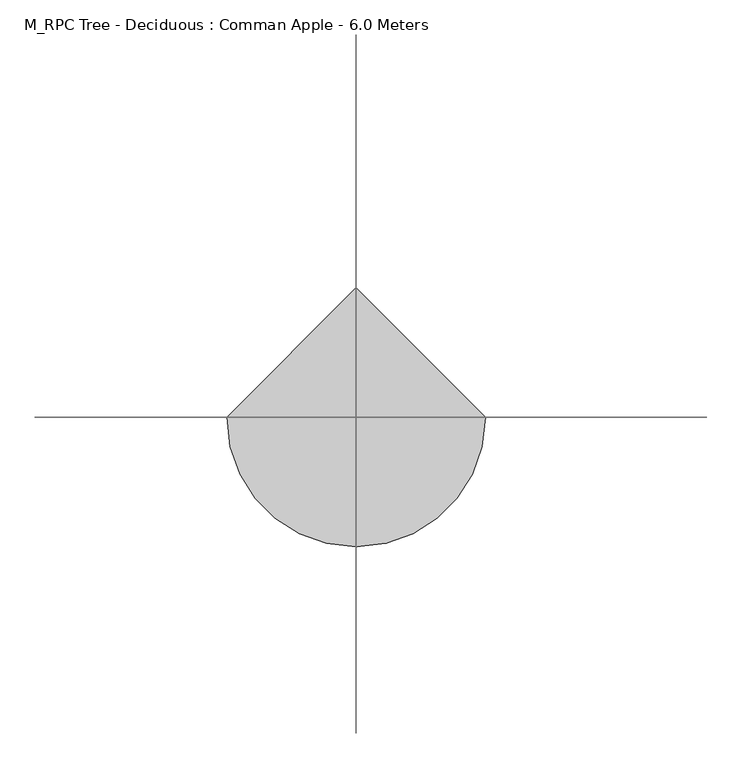
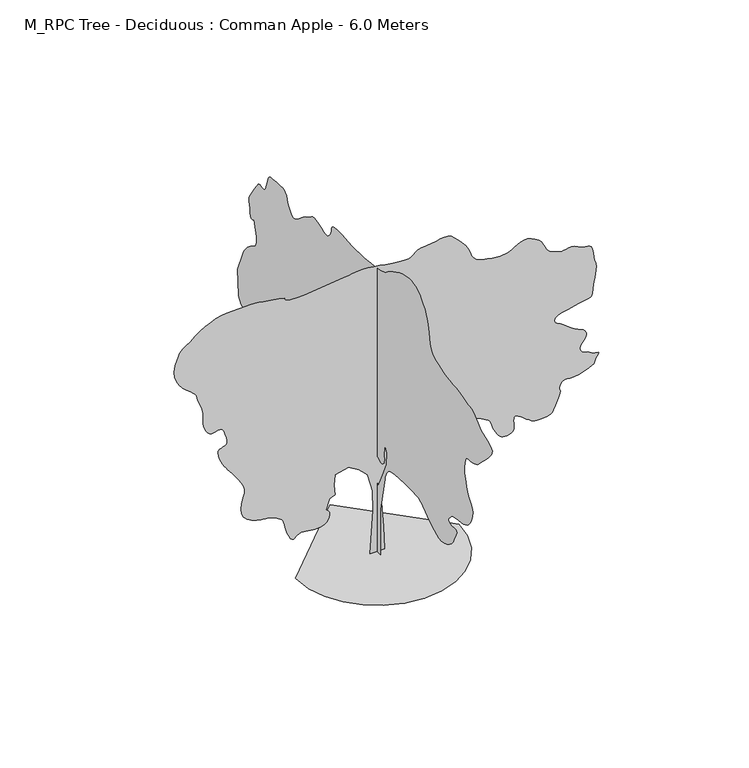
"""IFC4 building model written with IfcOpenShell, lengths in millimetres: geographic element geometry, M_RPC Tree - Deciduous : Comman Apple - 6.0 Meters."""

from ifc_helpers import new_model, si_unit, origin, place, context, project, spatial, triangles, source, transform, mapped, element, save


def m_rpc_tree_deciduous_comman_apple_6_0_meters_a7a636f8(model_context):
    return source(origin(), model_context, "Body", "Tessellation", [
        triangles([(-6.51e-05, -105.0228319, 0.0074776), (-6.15e-05, 138.9131143, 0.0074703), (-4.84e-05, 99.8833291, 458.6078719), (-3.14e-05, 129.1556067, 1014.7807915), (-1.8e-05, 226.7299288, 1414.8361691), (-8.5e-06, 392.6053236, 1649.0138809), (-1.1e-06, 577.9979682, 1805.1340027), (2.6e-06, 753.6305981, 1844.161417), (3.5e-06, 948.7807503, 1775.8613708), (1.5e-06, 1007.3257959, 1678.2863674), (-4e-06, 890.2357046, 1551.4387321), (-8.4e-06, 929.2657351, 1385.5635372), (-1.44e-05, 1153.685903, 1073.3258371), (-1.47e-05, 1543.9836639, 868.4182137), (-8.5e-06, 2109.9142365, 790.3606236), (7.6e-06, 2451.4244957, 1161.1408985), (2.53e-05, 2802.702182, 1580.7112186), (3.2e-05, 3349.1025513, 1531.9237896), (3.84e-05, 3544.2528488, 1649.0138809), (4.53e-05, 3534.5028625, 1883.1914474), (4.5e-05, 3358.8778267, 1961.2515083), (4.95e-05, 3232.0277206, 2175.9142776), (5.43e-05, 3534.5028625, 2185.6716763), (5.98e-05, 4139.453437, 2068.584201), (6.19e-05, 4208.0283211, 2104.1717091), (6.39e-05, 4273.9283684, 2140.0141434), (6.59e-05, 4334.553447, 2176.3691917), (6.78e-05, 4387.2284294, 2213.4942513), (6.96e-05, 4429.328476, 2251.6417774), (7.12e-05, 4458.2034576, 2291.0693127), (7.26e-05, 4471.2035362, 2332.0343994), (8.79e-05, 4500.4784935, 2829.6522812), (9.79e-05, 4334.6034439, 3249.2275429), (9.86e-05, 4317.5033249, 3282.3275574), (9.94e-05, 4292.2284142, 3321.5527794), (0.0001002, 4260.1033401, 3364.7027618), (0.000101, 4222.5283081, 3409.5526405), (0.0001017, 4180.8532356, 3453.9028404), (0.0001023, 4136.4533295, 3495.527916), (0.0001027, 4090.6782166, 3532.2027122), (0.0001029, 4046.5782921, 3560.9279938), (0.0001029, 4006.7531067, 3582.8278198), (0.000103, 3971.8782005, 3601.8278229), (0.0001031, 3942.6282417, 3621.8527634), (0.0001036, 3919.7031876, 3646.8529816), (0.0001043, 3903.7779968, 3680.7029503), (0.0001056, 3895.5282097, 3727.3530098), (0.0001072, 3894.4779831, 3782.2781456), (0.0001089, 3899.0529945, 3838.2279282), (0.0001108, 3908.3280098, 3895.0532387), (0.0001127, 3921.3530869, 3952.5282188), (0.0001147, 3937.2032822, 4010.528167), (0.0001167, 3954.9280724, 4068.8783844), (0.0001187, 3973.5780968, 4127.4033005), (0.0001184, 3998.5533165, 4107.2783661), (0.0001184, 4022.8532867, 4091.9531387), (0.0001185, 4045.7783409, 4086.1782005), (0.0001191, 4066.6532295, 4094.7532585), (0.0001202, 4084.8032845, 4122.4283134), (0.0001219, 4099.5532562, 4174.003363), (0.0001245, 4110.1781891, 4254.2534065), (0.000127, 4120.6784203, 4333.2285278), (0.0001287, 4132.0283089, 4385.4035408), (0.0001299, 4139.1281662, 4422.2036201), (0.0001309, 4136.8033081, 4455.0786484), (0.0001318, 4120.0031708, 4495.478508), (0.0001331, 4083.5533607, 4554.8286644), (0.0001348, 4022.3783157, 4644.5537109), (0.0001367, 3956.5782623, 4741.1289207), (0.0001382, 3906.9780922, 4815.003772), (0.0001392, 3869.5280525, 4868.5789902), (0.0001398, 3840.0781059, 4904.2041412), (0.0001401, 3814.5529198, 4924.3290756), (0.0001399, 3788.8780334, 4931.3042313), (0.0001393, 3758.9281174, 4927.5038818), (0.0001386, 3727.67799, 4918.0288788), (0.0001379, 3700.2029228, 4909.0788437), (0.0001374, 3675.45298, 4904.7291092), (0.0001372, 3652.4029335, 4909.0788437), (0.0001374, 3630.0528442, 4926.2289597), (0.000138, 3607.3527763, 4960.2792068), (0.0001393, 3583.2777924, 5015.3287537), (0.0001409, 3562.2279144, 5079.6288986), (0.0001424, 3546.3027237, 5137.7538391), (0.0001437, 3531.0527824, 5188.4042358), (0.0001447, 3512.0527794, 5230.1540131), (0.0001452, 3484.8526955, 5261.6794144), (0.0001452, 3445.0278008, 5281.604361), (0.0001446, 3388.1277855, 5288.5295197), (0.0001436, 3319.3276245, 5291.5793335), (0.0001428, 3248.6275795, 5298.5544891), (0.000142, 3178.9774704, 5306.2040222), (0.0001411, 3113.2274139, 5311.3042923), (0.0001402, 3054.3025223, 5310.5793365), (0.0001392, 3005.1273262, 5300.8293503), (0.000138, 2968.5772316, 5278.778952), (0.0001369, 2944.7272339, 5253.1543533), (0.0001361, 2929.602285, 5232.6294434), (0.0001354, 2919.9272942, 5214.0044174), (0.0001347, 2912.4774582, 5194.003894), (0.0001338, 2904.0023941, 5169.4042328), (0.0001326, 2891.2523003, 5136.9288895), (0.000131, 2871.0023735, 5093.3792221), (0.0001292, 2844.6522377, 5045.379245), (0.0001275, 2815.5772682, 5003.1539154), (0.000126, 2783.4271957, 4968.9542587), (0.0001248, 2747.8773308, 4945.0039764), (0.0001238, 2708.5521149, 4933.504097), (0.0001233, 2665.1521477, 4936.7039017), (0.0001232, 2617.3021614, 4956.7788391), (0.0001234, 2569.6771614, 4988.2542435), (0.0001238, 2525.4769524, 5023.3038483), (0.0001243, 2482.1194244, 5060.7288895), (0.0001247, 2437.0593842, 5099.3538574), (0.0001252, 2387.7318718, 5138.0038239), (0.0001254, 2331.5768692, 5175.4288651), (0.0001255, 2266.0343582, 5210.4790512), (0.0001256, 2205.0142456, 5244.5542969), (0.0001259, 2159.0142918, 5277.6040237), (0.0001262, 2120.3541515, 5306.2290207), (0.0001262, 2081.3542065, 5327.0044968), (0.0001258, 2034.3291698, 5336.5044983), (0.0001247, 1971.6040741, 5331.3292328), (0.0001227, 1885.4940685, 5308.0544907), (0.0001205, 1797.391452, 5276.8540695), (0.0001188, 1730.2863911, 5251.9544266), (0.0001175, 1678.8813892, 5236.1042313), (0.0001168, 1637.8888332, 5232.0288986), (0.0001166, 1602.0163136, 5242.4794235), (0.0001169, 1565.9737461, 5270.1544785), (0.0001177, 1524.4687214, 5317.8044769), (0.0001188, 1490.9861721, 5373.8045471), (0.0001201, 1475.2561729, 5423.9793915), (0.0001212, 1466.3511932, 5467.3296524), (0.0001221, 1453.3511147, 5502.8292297), (0.0001225, 1425.3286972, 5529.4543488), (0.0001222, 1371.366148, 5546.1794907), (0.000121, 1280.5334656, 5551.979718), (0.0001195, 1182.4759335, 5550.8792038), (0.0001183, 1108.9958982, 5547.8793869), (0.0001174, 1052.4133781, 5543.5296524), (0.0001165, 1005.0483187, 5538.3293884), (0.0001156, 959.220738, 5532.7791458), (0.0001147, 907.2482563, 5527.4044739), (0.0001136, 841.4482029, 5522.7041794), (0.0001125, 772.3506037, 5519.7043625), (0.0001115, 711.6155754, 5518.9044113), (0.0001107, 653.2705175, 5520.154335), (0.0001099, 591.3404677, 5523.2791443), (0.000109, 519.8504273, 5528.1294296), (0.0001078, 432.8303392, 5534.5046219), (0.0001065, 324.3052774, 5542.2291504), (0.000105, 203.687658, 5552.8796631), (0.0001037, 86.9965703, 5567.6043457), (0.0001026, -21.8426915, 5585.7544006), (0.0001018, -118.9050968, 5606.6292892), (0.0001012, -200.2644113, 5629.5546341), (0.0001011, -261.9952181, 5653.8543137), (0.0001012, -300.1702317, 5678.8295334), (0.0001016, -342.4727732, 5713.0297714), (0.000102, -413.9603428, 5761.2297363), (0.0001023, -506.7854181, 5817.0798157), (0.0001024, -613.0929554, 5874.3298096), (0.0001023, -725.0330704, 5926.6045258), (0.0001019, -834.75319, 5967.6299286), (0.0001011, -934.4057556, 5991.07966), (0.0001, -1022.9033335, 5999.8047089), (9.88e-05, -1104.7484104, 6000.0046967), (9.74e-05, -1180.4459702, 5990.3047073), (9.57e-05, -1250.5110249, 5969.3298248), (9.38e-05, -1315.4560432, 5935.7295502), (9.14e-05, -1375.7936394, 5888.1545471), (8.87e-05, -1432.0336658, 5825.2049011), (8.63e-05, -1478.7161362, 5768.8048553), (8.48e-05, -1512.7687088, 5733.7546692), (8.36e-05, -1538.2837212, 5707.9295013), (8.25e-05, -1559.3636845, 5679.2045105), (8.09e-05, -1580.1012268, 5635.454274), (7.84e-05, -1604.5962433, 5564.5545319), (7.46e-05, -1636.941362, 5454.4042786), (7.05e-05, -1667.1512913, 5330.3292938), (6.7e-05, -1688.656374, 5223.97939), (6.39e-05, -1710.6739254, 5132.8541382), (6.11e-05, -1742.4214062, 5054.3292801), (5.83e-05, -1793.1164223, 4985.8788071), (5.53e-05, -1871.9714928, 4924.9540375), (5.19e-05, -1988.2065491, 4868.9789658), (4.87e-05, -2119.0091755, 4825.5040031), (4.62e-05, -2237.6917568, 4799.6038399), (4.41e-05, -2347.6668755, 4784.9788605), (4.22e-05, -2452.3543808, 4775.3288681), (4.04e-05, -2555.1521759, 4764.2786705), (3.83e-05, -2659.5022018, 4745.5539413), (3.57e-05, -2768.8022163, 4712.8539024), (3.33e-05, -2866.4523605, 4683.5786545), (3.19e-05, -2939.5522591, 4672.2287659), (3.09e-05, -2996.927536, 4668.05373), (2.99e-05, -3047.4773575, 4660.2786232), (2.85e-05, -3100.0773445, 4638.1788094), (2.61e-05, -3163.6025368, 4590.9787834), (2.24e-05, -3246.9276833, 4507.9536186), (1.83e-05, -3354.9527756, 4422.0536293), (1.48e-05, -3474.4277504, 4364.503363), (1.18e-05, -3586.9278603, 4321.8033531), (9.3e-06, -3673.9780701, 4280.47855), (7e-06, -3717.153051, 4227.0283241), (5e-06, -3698.0280556, 4147.9782074), (2.9e-06, -3598.177755, 4029.8281517), (1.1e-06, -3473.4528099, 3906.2781349), (-3e-07, -3385.2276718, 3815.6781418), (-1.3e-06, -3323.4776619, 3751.5279877), (-1.9e-06, -3278.1025246, 3707.3530678), (-2.2e-06, -3239.0275841, 3676.6529068), (-2.3e-06, -3196.2275803, 3652.9528999), (-2.1e-06, -3139.5775497, 3629.777861), (-1.7e-06, -3075.1774109, 3613.37799), (-9e-07, -3016.2275208, 3608.6029907), (-2e-07, -2963.4272552, 3606.7278145), (2e-07, -2917.4774437, 3599.0529922), (2e-07, -2879.0021759, 3576.8528938), (-7e-07, -2848.7272797, 3531.452758), (-2.7e-06, -2827.3521309, 3454.1278267), (-5.1e-06, -2815.7522575, 3369.9277336), (-7e-06, -2813.3521133, 3305.0276253), (-8.6e-06, -2818.6523712, 3252.4026398), (-1.02e-05, -2830.0772552, 3205.052623), (-1.19e-05, -2846.1271477, 3156.0024193), (-1.39e-05, -2865.2274353, 3098.2524559), (-1.64e-05, -2885.9023361, 3024.8022881), (-1.92e-05, -2914.627327, 2946.6774055), (-2.18e-05, -2954.4522217, 2877.5772629), (-2.43e-05, -2998.5524368, 2814.6273262), (-2.67e-05, -3040.0775185, 2754.9021927), (-2.9e-05, -3072.2275909, 2695.5270378), (-3.11e-05, -3088.152491, 2633.6020386), (-3.3e-05, -3081.052343, 2566.2020828), (-3.46e-05, -3060.4274391, 2500.277037), (-3.6e-05, -3039.1022873, 2443.7194427), (-3.71e-05, -3015.2522896, 2395.18694), (-3.79e-05, -2986.9272743, 2353.3118797), (-3.85e-05, -2952.3273514, 2316.7293743), (-3.88e-05, -2909.5023491, 2284.0717747), (-3.89e-05, -2856.6273788, 2253.9743385), (-3.87e-05, -2791.7272705, 2230.5618141), (-3.8e-05, -2717.452153, 2216.0268002), (-3.71e-05, -2638.7520149, 2206.0967377), (-3.62e-05, -2560.5271385, 2196.5117123), (-3.56e-05, -2487.799601, 2182.9993103), (-3.53e-05, -2425.47201, 2161.2942398), (-3.56e-05, -2378.5043827, 2127.129174), (-3.62e-05, -2345.7043499, 2089.8041267), (-3.68e-05, -2322.8042942, 2060.3341232), (-3.73e-05, -2310.1443111, 2037.0066227), (-3.78e-05, -2308.0692924, 2018.1191128), (-3.84e-05, -2316.9168629, 2001.9616688), (-3.92e-05, -2337.029298, 1986.8265461), (-4.01e-05, -2368.7468388, 1971.0090523), (-4.1e-05, -2411.2468609, 1962.5040482), (-4.16e-05, -2459.0394379, 1965.0915356), (-4.21e-05, -2505.4770103, 1970.754126), (-4.27e-05, -2543.876992, 1971.4641117), (-4.34e-05, -2567.6019974, 1959.2041042), (-4.44e-05, -2569.9771431, 1925.949012), (-4.59e-05, -2544.3769615, 1863.6765049), (-4.75e-05, -2509.7520401, 1792.5014889), (-4.89e-05, -2484.8695473, 1735.1513557), (-4.99e-05, -2462.7095627, 1687.5312973), (-5.08e-05, -2436.2819607, 1645.5437439), (-5.14e-05, -2398.5893486, 1605.0912712), (-5.19e-05, -2342.631863, 1562.0787804), (-5.22e-05, -2261.4142914, 1512.4087017), (-5.2e-05, -2169.1316975, 1473.3237328), (-5.1e-05, -2083.5066914, 1461.3762062), (-4.95e-05, -2002.8290577, 1471.4462311), (-4.76e-05, -1925.3965748, 1498.4137711), (-4.53e-05, -1849.4990273, 1537.1587898), (-4.28e-05, -1773.4289612, 1582.5612511), (-4.02e-05, -1695.4838642, 1629.498793), (-3.77e-05, -1622.0062271, 1676.8063705), (-3.54e-05, -1558.0836754, 1724.7963192), (-3.31e-05, -1500.136195, 1770.5689613), (-3.11e-05, -1444.578685, 1811.2214218), (-2.93e-05, -1387.8260445, 1843.8489361), (-2.77e-05, -1326.2960793, 1865.5564774), (-2.64e-05, -1256.4010723, 1873.4340488), (-2.5e-05, -1159.1384045, 1874.2889385), (-2.3e-05, -1027.910804, 1875.4840691), (-2.07e-05, -877.7382116, 1874.971455), (-1.86e-05, -723.6380974, 1870.7039829), (-1.67e-05, -580.6329818, 1860.6339581), (-1.55e-05, -463.7428782, 1842.7115055), (-1.52e-05, -387.9878002, 1814.8914013), (-1.57e-05, -343.2127716, 1776.8839828), (-1.66e-05, -308.1652379, 1730.6863667), (-1.77e-05, -281.2252217, 1677.6614056), (-1.92e-05, -260.7727092, 1619.1738419), (-2.08e-05, -245.1829449, 1556.5887085), (-2.26e-05, -232.8366782, 1491.2736546), (-2.44e-05, -222.1121693, 1424.5935677), (-3.85e-05, -114.7803395, 897.6907001), (-2.01e-05, -26.9632706, 1297.7460777), (-1.3e-05, -173.3248856, 1609.9838505), (-6.5e-06, -300.1727388, 1892.9489914), (2e-07, -319.6852469, 2127.129174), (4.7e-06, -251.3852008, 2244.2167946), (-4e-07, -222.1119331, 2058.8266571), (-1.7e-06, -228.0859325, 2017.1790539), (-3e-06, -232.2679447, 1976.5565334), (-4.1e-06, -232.865183, 1937.9815624), (-5.1e-06, -228.0859325, 1902.4790783), (-5.9e-06, -216.1379155, 1871.0740185), (-6.4e-06, -195.2293988, 1844.788995), (-6.5e-06, -163.5673779, 1824.6489452), (-6.1e-06, -127.1833524, 1819.4714996), (-5.2e-06, -93.5303284, 1831.0189053), (-4.2e-06, -62.949051, 1849.7389835), (-3.3e-06, -35.7820297, 1866.0664753), (-2.9e-06, -12.3698845, 1870.4490566), (-3.1e-06, 6.9458055, 1853.3239391), (-4.3e-06, 21.8237678, 1805.1340027), (-6.1e-06, 32.3777748, 1741.0688725), (-7.7e-06, 39.3472803, 1682.1263947), (-9.3e-06, 43.330036, 1627.4512436), (-1.08e-05, 44.9230347, 1576.1888203), (-1.22e-05, 44.724037, 1527.4862698), (-1.37e-05, 43.330036, 1480.4911732), (-1.51e-05, 41.3385332, 1434.3511116), (137.391859, 0.0003253, 0.0), (-133.3141101, 0.0003334, 0.0), (-73.1573078, 0.0002372, 832.1731876), (-83.1833128, 0.0002433, 1223.1935062), (-183.4456522, 0.0001982, 1574.1087147), (-333.8377625, 0.0002049, 1724.5014244), (-534.3604428, 0.0002126, 1844.8164642), (-785.015601, 0.0002192, 1784.6589443), (-805.0681561, 0.0002168, 1584.1363003), (-785.015601, 0.0002134, 1393.6386257), (-885.278231, 0.0002156, 1343.5060753), (-955.4607931, 0.0002149, 1153.0084007), (-936.3432827, 0.0002675, 1139.8859459), (-918.5407356, 0.0002668, 1125.3558735), (-903.3707314, 0.0002661, 1108.0233559), (-892.1456898, 0.0002654, 1086.4808481), (-886.1831903, 0.0002648, 1059.3258196), (-886.7981964, 0.0002643, 1025.1533415), (-895.3032005, 0.0002639, 982.565752), (-913.9532249, 0.0002639, 940.0632591), (-942.5982788, 0.0002642, 906.5057144), (-978.963283, 0.0002649, 881.0181713), (-1020.7633478, 0.0002659, 862.7181982), (-1065.71838, 0.0002671, 850.7331739), (-1111.553373, 0.0002683, 844.1856812), (-1155.9834372, 0.0002696, 842.1981571), (-1199.4784567, 0.000271, 844.8881819), (-1243.6759769, 0.0002724, 851.4356747), (-1288.0485592, 0.0002738, 859.5631582), (-1332.0685467, 0.0002752, 866.9856703), (-1375.2135876, 0.0002766, 871.4282043), (-1416.9560978, 0.0002778, 870.610667), (-1456.7686386, 0.0002789, 862.2507122), (-1490.9986713, 0.0002796, 844.3906832), (-1518.2137253, 0.0002801, 821.2681847), (-1541.2187164, 0.0002805, 799.9006662), (-1562.8187061, 0.0002809, 787.3031067), (-1585.8236973, 0.0002817, 790.4881594), (-1613.0387512, 0.0002829, 816.475672), (-1647.2663132, 0.0002313, 872.2782251), (-1679.7413658, 0.0002334, 944.3882858), (-1702.0463997, 0.0002351, 1013.3457773), (-1717.508828, 0.0002365, 1077.2133905), (-1729.4639122, 0.0002377, 1134.0684231), (-1741.2438618, 0.0002387, 1181.9784348), (-1756.1814674, 0.0002397, 1219.0134562), (-1777.6064678, 0.0002407, 1243.2460613), (-1804.2939377, 0.0002418, 1262.5659576), (-1833.963929, 0.000243, 1284.8709915), (-1868.368951, 0.0002444, 1308.2261066), (-1909.2639839, 0.000246, 1330.7035137), (-1958.3990662, 0.0002477, 1350.3761501), (-2017.5341194, 0.0002497, 1365.3136105), (-2088.4191822, 0.0002519, 1373.5860706), (-2170.7616852, 0.0002011, 1382.5010788), (-2258.5417923, 0.000204, 1401.9385551), (-2344.9193687, 0.0002071, 1433.8310852), (-2423.054425, 0.0002101, 1480.1036968), (-2486.1043556, 0.0002129, 1542.6862141), (-2527.2271362, 0.0002153, 1623.5087517), (-2539.6019623, 0.0002172, 1724.5014244), (-2528.5270569, 0.0002183, 1822.2489464), (-2508.6771057, 0.0002189, 1897.5490013), (-2487.2420769, 0.0002192, 1958.6416386), (-2471.4293793, 0.0001661, 2013.7690876), (-2468.4170631, 0.0001669, 2071.1791008), (-2485.3994568, 0.0001684, 2139.1117275), (-2529.5769928, 0.000171, 2225.8093426), (-2588.3771828, 0.0001741, 2318.6767845), (-2644.0269836, 0.000177, 2400.3194756), (-2695.8270195, 0.0001796, 2471.7869156), (-2743.0773331, 0.000182, 2534.1270058), (-2785.0520966, 0.0001306, 2588.4271797), (-2821.0522247, 0.0001324, 2635.6772026), (-2850.4021774, 0.0001339, 2676.9770073), (-2878.5522034, 0.0001354, 2723.8270546), (-2908.6274025, 0.0001372, 2782.7522369), (-2936.4274498, 0.000139, 2847.4523575), (-2957.7523109, 0.0001406, 2911.6522179), (-2968.3522453, 0.0001418, 2969.0024963), (-2964.0525078, 0.0001423, 3013.2024147), (-2940.6524826, 0.000142, 3037.927359), (-2905.0023331, 0.0001411, 3050.052491), (-2869.2021927, 0.0001402, 3062.5523094), (-2836.72714, 0.0001395, 3078.1775185), (-2811.1022507, 0.000139, 3099.7773628), (-2795.8023125, 0.000139, 3130.1525436), (-2794.3771088, 0.0001396, 3172.1025993), (-2810.3022995, 0.0001409, 3228.4276497), (-2831.7271545, 8.9e-05, 3286.3526024), (-2846.6774048, 9.02e-05, 3332.2027107), (-2858.4522675, 9.1e-05, 3367.3276016), (-2870.4024101, 9.18e-05, 3393.1777679), (-2885.8523392, 9.25e-05, 3411.1278351), (-2908.17743, 9.33e-05, 3422.5777176), (-2940.6524826, 9.44e-05, 3428.9526192), (-2978.7524826, 9.55e-05, 3427.0527351), (-3016.0025345, 9.65e-05, 3417.4277412), (-3052.7023293, 9.74e-05, 3407.1277885), (-3089.2524239, 9.85e-05, 3403.1027435), (-3125.9775078, 9.97e-05, 3412.4277557), (-3163.2025612, 0.0001012, 3442.1026886), (-3201.3275597, 0.0001032, 3499.1276962), (-3229.5025841, 0.0001051, 3569.6277534), (-3241.3777313, 0.0001065, 3637.1529922), (-3243.9525742, 0.0001076, 3704.8529297), (-3244.2275574, 0.0001086, 3775.9029533), (-3249.2525414, 5.65e-05, 3853.4031647), (-3266.0276802, 5.83e-05, 3940.5780762), (-3301.5775452, 6.09e-05, 4040.5533691), (-3337.877655, 6.33e-05, 4130.928376), (-3357.5276184, 6.48e-05, 4192.7283829), (-3368.4028267, 6.58e-05, 4234.1784691), (-3378.4027977, 6.65e-05, 4263.5284218), (-3395.4276306, 6.74e-05, 4289.0033203), (-3427.3277184, 6.88e-05, 4318.8785316), (-3482.0528664, 7.1e-05, 4361.3785538), (-3552.8529053, 2.06e-05, 4417.8785934), (-3623.6529442, 2.37e-05, 4484.3786041), (-3688.3030678, 2.68e-05, 4561.0535751), (-3740.6780685, 2.96e-05, 4648.0787865), (-3774.6530296, 3.21e-05, 4745.6289368), (-3784.0780357, 3.4e-05, 4853.8540169), (-3762.7778824, 3.51e-05, 4972.9790131), (-3729.8778557, -1.77e-05, 5076.7040771), (-3704.502951, -1.74e-05, 5145.8539261), (-3680.7029503, -1.74e-05, 5191.3290573), (-3652.5279259, -1.78e-05, 5224.0043884), (-3614.0029518, -1.85e-05, 5254.7792542), (-3559.1778099, -1.95e-05, 5294.454158), (-3482.0528664, -2.09e-05, 5353.9790131), (-3391.1775993, -2.26e-05, 5424.8793365), (-3298.9027084, -2.44e-05, 5490.3794083), (-3205.0276245, -2.63e-05, 5548.6543396), (-3109.4273552, -2.84e-05, 5598.0042343), (-3011.8774956, -3.07e-05, 5636.6297836), (-2912.2274734, -3.33e-05, 5662.8293472), (-2810.3022995, -3.62e-05, 5674.8047791), (-2339.0719059, -5.01e-05, 5684.8297485), (-2273.3618179, -5.21e-05, 5682.2043274), (-2197.6542297, -5.44e-05, 5674.854776), (-2113.614156, -3.7e-06, 5663.5293045), (-2022.9115528, -6.6e-06, 5649.0546066), (-1927.2115803, -9.7e-06, 5632.2294708), (-1828.1764915, -1.3e-05, 5613.8044327), (-1727.4763882, -1.63e-05, 5594.6044418), (-1724.3188774, -1.66e-05, 5575.4544479), (-1715.1112999, -1.72e-05, 5557.4543839), (-1693.8014088, -1.8e-05, 5541.7291809), (-1654.3413174, -1.94e-05, 5529.4293503), (-1590.6763081, -2.14e-05, 5521.6792419), (-1496.7561687, -2.42e-05, 5519.6293671), (-1366.5335941, -2.81e-05, 5524.4296555), (-604.5454757, -4.94e-05, 5614.6543808), (-529.8304141, -5.15e-05, 5621.554541), (-464.7628741, 1e-07, 5631.7794983), (-403.0278342, -1.6e-06, 5642.554422), (-338.3102729, -3.4e-06, 5651.0294861), (-264.297712, -5.6e-06, 5654.4042801), (-174.6758932, -8.3e-06, 5649.9045547), (-63.1312982, -1.19e-05, 5634.7043198), (53.8502923, -1.57e-05, 5614.4793915), (156.9766284, -1.9e-05, 5596.879303), (248.3524462, -2.19e-05, 5582.1046234), (330.0827591, -2.45e-05, 5570.2791824), (404.2703093, -2.69e-05, 5561.6297104), (473.0203643, -2.9e-05, 5556.304454), (538.4379192, -3.1e-05, 5554.5045639), (593.7429737, -3.25e-05, 5562.8296371), (635.895488, -3.35e-05, 5584.3044891), (672.6080727, -3.41e-05, 5613.6794403), (711.6030762, -3.48e-05, 5645.7042297), (760.5931091, -3.58e-05, 5675.0797623), (827.2981945, -3.75e-05, 5696.5546143), (919.4332684, -4.01e-05, 5704.904686), (1019.3733164, -4.3e-05, 5711.6048584), (1106.3358862, -4.54e-05, 5726.7545151), (1183.3009558, -4.74e-05, 5742.7796997), (1253.2485031, -4.94e-05, 5752.1297104), (1319.1659912, -5.14e-05, 5747.279425), (1384.0286018, -5.37e-05, 5720.6793045), (1450.8211819, -3.2e-06, 5664.7798096), (1514.7787605, -6.1e-06, 5597.4042709), (1569.6162563, -8.6e-06, 5539.5043167), (1616.0337719, -1.07e-05, 5488.254538), (1654.7363514, -1.26e-05, 5440.8795227), (1686.421336, -1.42e-05, 5394.5544434), (1711.7939152, -1.57e-05, 5346.4544724), (1731.5539009, -1.7e-05, 5293.8291962), (1749.3263626, -1.84e-05, 5241.0039322), (1770.606459, -1.97e-05, 5194.1538849), (1798.9013889, -2.12e-05, 5153.0790665), (1837.7189323, 3.06e-05, 5117.6039063), (1890.5690495, 2.85e-05, 5087.6039932), (1960.9566135, 2.61e-05, 5062.8287613), (2052.3915848, 2.3e-05, 5043.1537994), (2147.2741653, 2e-05, 5028.9540848), (2227.0742363, 1.75e-05, 5020.3540283), (2293.8969017, 1.55e-05, 5016.8542419), (2349.8443588, 1.38e-05, 5017.9041779), (2397.0244732, 1.25e-05, 5023.0038666), (2437.5369713, 1.14e-05, 5031.5789246), (2473.4920441, 1.05e-05, 5043.1537994), (2512.0269012, 9.7e-06, 5063.479303), (2558.2519867, 8.7e-06, 5093.9791855), (2611.3522339, 7.6e-06, 5127.6038773), (2670.3771194, 6.3e-06, 5157.4043839), (2734.5272736, 4.7e-06, 5176.304393), (2802.8521729, 2.7e-06, 5177.3293304), (2874.5271584, 2e-07, 5153.4540436), (2937.3023964, -2.2e-06, 5120.2293274), (2982.5272522, -3.9e-06, 5095.0541199), (3014.7523201, -5.2e-06, 5073.7292587), (3038.5773193, -6.2e-06, 5052.0788361), (3058.5525536, -7.2e-06, 5025.854274), (3079.2024559, -8.3e-06, 4990.8790833), (3105.1276176, -9.8e-06, 4942.9041046), (3132.7273865, 4.2e-05, 4892.8036743), (3157.7026062, 4.07e-05, 4852.7037964), (3183.5274834, 3.94e-05, 4820.3037392), (3213.7526733, 3.81e-05, 4793.3539307), (3251.8776718, 3.66e-05, 4769.5539299), (3301.4025558, 3.48e-05, 4746.6538742), (3365.8276932, 3.25e-05, 4722.3289055), (3431.1277771, 3.03e-05, 4707.5036476), (3484.3277275, 2.88e-05, 4709.3538254), (3530.502816, 2.76e-05, 4719.9537598), (3574.7527313, 2.64e-05, 4731.4539299), (3622.1780342, 2.51e-05, 4735.9286568), (3677.8278351, 2.33e-05, 4725.4787132), (3746.8029854, 2.07e-05, 4692.2537064), (3818.1279922, 1.81e-05, 4658.4537346), (3877.8781242, 1.61e-05, 4644.1287369), (3926.7530479, 1.45e-05, 4638.053817), (3965.453302, 1.32e-05, 4629.003788), (3994.7032608, 1.2e-05, 4605.7287552), (4015.1531754, 6.41e-05, 4557.0285301), (4027.5532906, 6.24e-05, 4471.6785072), (4039.2031609, 6.08e-05, 4384.4785973), (4054.5533867, 5.95e-05, 4327.8035683), (4069.9033218, 5.84e-05, 4286.7284592), (4081.5781906, 5.75e-05, 4246.3533073), (4085.8532204, 5.65e-05, 4191.7784409), (4079.1033417, 5.55e-05, 4108.1033157), (4057.628199, 5.42e-05, 3980.3782631), (4035.5280945, 0.0001063, 3847.1779633), (4024.4781876, 0.0001052, 3752.0279572), (4017.103347, 0.0001045, 3687.5778214), (4006.0531494, 0.0001042, 3646.453006), (3983.9530449, 0.0001045, 3621.2777985), (3943.4531914, 0.0001054, 3604.7279366), (3877.1531685, 0.0001072, 3589.3780014), (3783.9280449, 0.0001097, 3571.4279343), (3675.2779907, 0.0001126, 3551.3777046), (3562.7778809, 0.0001156, 3528.3279488), (3457.9778824, 0.0001183, 3501.452845), (3372.477578, 0.0001204, 3469.8277405), (3317.8527145, 0.0001215, 3432.5776886), (3305.6525871, 0.0001212, 3388.8527412), (3318.4276794, 0.0001203, 3351.9776665), (3332.9526649, 0.0001195, 3330.9027901), (3352.2276512, 0.0001188, 3318.0777008), (3379.2027489, 0.0001178, 3305.9525688), (3416.8777748, 0.0001164, 3286.9775642), (3468.2528366, 0.0001143, 3253.627565), (3536.2527557, 0.0001115, 3198.3524506), (3611.5028137, 0.0001084, 3139.7525391), (3681.477903, 0.0001057, 3097.8024834), (3744.6281181, 0.0001033, 3067.0773239), (3799.3529755, 0.0001547, 3042.1273933), (3844.053154, 0.000153, 3017.5524399), (3877.2031654, 0.0001516, 2987.877507), (3897.2031075, 0.0001504, 2947.702343), (3897.9280632, 0.0001497, 2900.4773186), (3879.7280113, 0.0001495, 2853.6272713), (3850.6530418, 0.0001497, 2807.4771812), (3818.7529541, 0.00015, 2762.3773178), (3792.1281258, 0.0001501, 2718.6770782), (3778.8280655, 0.0001499, 2676.7270226), (3786.9281525, 0.0001491, 2636.8771294), (3809.6279297, 0.0001479, 2605.4770111), (3834.8031372, 0.0001469, 2585.8520462), (3862.4281952, 0.0001459, 2573.7522034), (3892.5031036, 0.0001448, 2564.9771576), (3925.0281532, 0.0001437, 2555.3271652), (3960.0280518, 0.0001425, 2540.6019012), (3997.4780914, 0.000141, 2516.5769142), (4036.1783455, 0.0001395, 2494.674472), (4072.603157, 0.0001383, 2485.0593613), (4103.2283226, 0.0001373, 2481.5793411), (4124.5531837, 0.0001366, 2478.1019371), (4133.1032433, 0.0001362, 2468.4845009), (4125.3284271, 0.0001895, 2446.5919418), (4097.7283676, 0.0001897, 2406.2819023), (4070.2033035, 0.0001899, 2361.9969601), (4057.9281807, 0.0001898, 2329.461882), (4050.3783508, 0.0001896, 2304.4693668), (4037.0532921, 0.0001897, 2282.8093517), (4007.403067, 0.0001903, 2260.2742447), (3950.9280258, 0.0001915, 2232.649332), (3857.1032295, 0.0001938, 2195.731818), (3751.1030136, 0.0001965, 2165.9741867), (3663.5278358, 0.000199, 2156.5616798), (3591.9278458, 0.0002011, 2158.3742146), (3533.8029053, 0.0002029, 2162.291708), (3486.7528702, 0.0002043, 2159.1942226), (3448.2778931, 0.0002051, 2139.9592049), (3415.9528313, 0.0002054, 2095.4691879), (3396.9028313, 0.0002053, 2048.9641777), (3394.8526657, 0.000205, 2022.9766651), (3402.2777939, 0.0002045, 2007.3391022), (3411.6278046, 0.000204, 1991.8765285), (3415.3778664, 0.0002035, 1966.4166), (3405.9528603, 0.0002031, 1920.7865364), (3375.8526627, 0.0002029, 1844.8164642), (3339.8025375, 0.0002027, 1759.2289558), (3313.4026955, 0.0002024, 1690.476321), (3290.3526489, 0.0002023, 1636.9838013), (3264.3024948, 0.0002025, 1597.1712605), (3228.9526176, 0.0002032, 1569.4613239), (3178.0025299, 0.0002044, 1552.2737103), (3105.1276176, 0.0002065, 1544.0311901), (3032.1274223, 0.0002086, 1540.6111954), (2980.1523972, 0.0002101, 1539.996262), (2942.0273987, 0.0002113, 1543.7687061), (2910.5772835, 0.0002124, 1553.5012516), (2878.6022003, 0.0002136, 1570.7762146), (2838.902298, 0.0002152, 1597.1712605), (2784.3021423, 0.0002174, 1634.2663799), (2725.2272598, 0.0002198, 1675.6263554), (2676.327047, 0.0002218, 1712.2539162), (2636.7271385, 0.0002234, 1741.8638821), (2605.5270081, 0.0002246, 1762.1813919), (2581.8769981, 0.0002254, 1770.9214108), (2564.9021622, 0.0002259, 1765.8038452), (2553.7019737, 0.0002259, 1744.5538342), (2547.3770691, 0.0002257, 1717.2514309), (2544.9269279, 0.0002254, 1694.3364052), (2545.2769066, 0.0002251, 1674.0488354), (2547.3770691, 0.0002247, 1654.6388283), (2550.2018967, 0.0002244, 1634.3538746), (2552.6520378, 0.0002239, 1611.4362328), (2553.7019737, 0.0002235, 1584.1363003), (2552.2770607, 0.0002231, 1554.2312943), (2547.1520828, 0.0002228, 1525.3811657), (2537.1271133, 0.0002227, 1498.6361412), (2520.9519379, 0.0002229, 1475.0461567), (2497.4295364, 0.0002233, 1455.666235), (2465.3044624, 0.000224, 1441.5461666), (2423.3594936, 0.0002251, 1433.7435905), (2380.6244568, 0.0002264, 1432.0761051), (2345.4293667, 0.0002275, 1436.3736626), (2315.4968914, 0.0002286, 1447.6861988), (2288.5467922, 0.0002297, 1467.0661205), (2262.2967957, 0.0002309, 1495.5661251), (2234.4692791, 0.0002323, 1534.2387646), (2202.7842945, 0.000234, 1584.1363003), (2173.4642818, 0.0002356, 1638.6213467), (2152.3892601, 0.0001837, 1689.7763638), (2136.7516972, 0.0001848, 1736.7213181), (2123.7442062, 0.0001858, 1778.5789375), (2110.561726, 0.0001868, 1814.4739849), (2094.3967243, 0.0001877, 1843.5290428), (2072.4441399, 0.0001886, 1864.8690193), (2041.9866966, 0.0001898, 1883.516573), (2003.1091278, 0.0001913, 1904.796524), (1957.2165802, 0.000193, 1928.2690739), (1905.7115845, 0.0001949, 1953.4966038), (1849.996526, 0.000197, 1980.0365536), (1791.4764061, 0.0001991, 2007.4565369), (1731.5539009, 0.0002013, 2035.3141388), (1390.663662, 0.0002115, 2035.3141388), (1200.1659874, 0.0002139, 1814.7364689), (1195.6959841, 0.0002136, 1784.6589443), (1190.1709579, 0.0002133, 1754.578949), (1182.5409731, 0.0002131, 1724.5014244), (1171.7559483, 0.0002129, 1694.4238998), (1156.7583899, 0.0002129, 1664.3437592), (1136.5033762, 0.0002131, 1634.2663799), (1109.9308702, 0.0002134, 1604.1888554), (1086.2834038, 0.0002138, 1578.7562508), (1071.7558748, 0.0002139, 1561.5687824), (1060.7358353, 0.0002141, 1551.0461689), (1047.610837, 0.0002144, 1545.6087101), (1026.7682865, 0.000215, 1543.6787407), (992.5982792, 0.000216, 1543.6787407), (939.4857508, 0.0002176, 1544.0311901), (873.0156801, 0.0002196, 1546.8661915), (804.2656614, 0.0002218, 1554.4362236), (735.8656214, 0.000224, 1565.3387558), (670.4455593, 0.0002262, 1578.1712574), (610.6404888, 0.0002281, 1591.5313431), (559.0754313, 0.0002299, 1604.0112499), (518.3879076, 0.0002312, 1614.2138248), (483.4279049, 0.0002324, 1624.5613037), (447.4153502, 0.0002337, 1638.0662933), (410.5253417, 0.000235, 1654.201355), (372.9353033, 0.0002364, 1672.4413754), (334.8177535, 0.0001845, 1692.2589157), (296.3502432, 0.0001859, 1713.1313335), (257.7052002, 0.0001874, 1734.5288647), (77.2350658, 0.0002405, 1353.5335155), (67.2090517, 0.0002365, 1062.7733562), (117.3398399, 0.0002792, 451.1778749), (-1522.7162121, 1.1e-06, 0.0098235), (-1482.4612564, -348.9052657, 0.0098339), (-1367.8136032, -669.3205553, 0.0098435), (-1187.9534334, -952.0632534, 0.0098519), (-952.0632534, -1187.9534334, 0.0098589), (-669.3205553, -1367.8136032, 0.0098643), (-348.9052657, -1482.4612564, 0.0098677), (6.66e-05, -1522.7162121, 0.0098689), (348.9052657, -1482.4612564, 0.0098677), (669.3205553, -1367.8136032, 0.0098643), (952.0632534, -1187.9534334, 0.0098589), (1187.9534334, -952.0632534, 0.0098519), (1367.8136032, -669.3205553, 0.0098435), (1482.4612564, -348.9052657, 0.0098339), (1522.7162121, 0.0001238, 0.0098235), (-0.0001997, 1522.7162121, 0.0097782)], [[300, 1, 301], [299, 300, 301], [299, 301, 302], [298, 299, 302], [297, 298, 302], [296, 297, 302], [296, 302, 303], [295, 296, 303], [294, 295, 303], [293, 294, 303], [292, 293, 303], [1, 2, 3], [301, 1, 3], [301, 3, 4], [301, 4, 5], [327, 301, 5], [326, 327, 5], [326, 5, 6], [325, 326, 6], [324, 325, 6], [323, 324, 6], [322, 323, 6], [321, 322, 6], [320, 321, 6], [19, 20, 21], [18, 19, 21], [17, 18, 21], [17, 21, 22], [320, 6, 7], [319, 320, 7], [291, 292, 303], [291, 303, 304], [290, 291, 304], [261, 262, 263], [260, 261, 263], [260, 263, 264], [259, 260, 264], [259, 264, 265], [258, 259, 265], [10, 11, 12], [14, 15, 16], [258, 265, 266], [257, 258, 266], [205, 206, 207], [204, 205, 207], [204, 207, 208], [203, 204, 208], [203, 208, 209], [202, 203, 209], [202, 209, 210], [257, 266, 267], [10, 12, 13], [257, 267, 268], [257, 268, 269], [256, 257, 269], [256, 269, 270], [256, 270, 271], [255, 256, 271], [255, 271, 272], [255, 272, 273], [255, 273, 274], [255, 274, 275], [255, 275, 276], [255, 276, 277], [254, 255, 277], [254, 277, 278], [254, 278, 279], [254, 279, 280], [253, 254, 280], [253, 280, 281], [253, 281, 282], [289, 290, 304], [10, 13, 14], [10, 14, 16], [10, 16, 17], [10, 17, 22], [9, 10, 22], [201, 202, 210], [201, 210, 211], [201, 211, 212], [201, 212, 213], [201, 213, 214], [201, 214, 215], [201, 215, 216], [201, 216, 217], [201, 217, 218], [201, 218, 219], [200, 201, 219], [199, 200, 219], [198, 199, 219], [197, 198, 219], [196, 197, 219], [195, 196, 219], [194, 195, 219], [194, 219, 220], [193, 194, 220], [192, 193, 220], [191, 192, 220], [190, 191, 220], [189, 190, 220], [189, 220, 221], [188, 189, 221], [252, 253, 282], [252, 282, 283], [188, 221, 222], [187, 188, 222], [251, 252, 283], [187, 222, 223], [23, 24, 25], [318, 319, 7], [56, 57, 58], [56, 58, 59], [55, 56, 59], [55, 59, 60], [54, 55, 60], [54, 60, 61], [54, 61, 62], [23, 25, 26], [186, 187, 223], [23, 26, 27], [23, 27, 28], [23, 28, 29], [23, 29, 30], [23, 30, 31], [23, 31, 32], [23, 32, 33], [23, 33, 34], [23, 34, 35], [23, 35, 36], [23, 36, 37], [23, 37, 38], [23, 38, 39], [23, 39, 40], [23, 40, 41], [23, 41, 42], [23, 42, 43], [23, 43, 44], [22, 23, 44], [22, 44, 45], [9, 22, 45], [9, 45, 46], [9, 46, 47], [9, 47, 48], [8, 9, 48], [8, 48, 49], [8, 49, 50], [8, 50, 51], [8, 51, 52], [8, 52, 53], [8, 53, 54], [250, 251, 283], [250, 283, 284], [288, 289, 304], [288, 304, 305], [186, 223, 224], [287, 288, 305], [313, 314, 315], [312, 313, 315], [311, 312, 315], [310, 311, 315], [310, 315, 316], [309, 310, 316], [308, 309, 316], [308, 316, 317], [307, 308, 317], [306, 307, 317], [306, 317, 318], [305, 306, 318], [305, 318, 7], [305, 7, 8], [305, 8, 54], [305, 54, 62], [305, 62, 63], [305, 63, 64], [305, 64, 65], [305, 65, 66], [305, 66, 67], [305, 67, 68], [305, 68, 69], [305, 69, 70], [305, 70, 71], [305, 71, 72], [305, 72, 73], [305, 73, 74], [305, 74, 75], [305, 75, 76], [305, 76, 77], [305, 77, 78], [305, 78, 79], [305, 79, 80], [305, 80, 81], [305, 81, 82], [305, 82, 83], [305, 83, 84], [305, 84, 85], [305, 85, 86], [305, 86, 87], [305, 87, 88], [305, 88, 89], [305, 89, 90], [305, 90, 91], [305, 91, 92], [134, 135, 136], [134, 136, 137], [133, 134, 137], [133, 137, 138], [132, 133, 138], [132, 138, 139], [132, 139, 140], [131, 132, 140], [131, 140, 141], [131, 141, 142], [131, 142, 143], [130, 131, 143], [130, 143, 144], [130, 144, 145], [286, 287, 305], [186, 224, 225], [185, 186, 225], [249, 250, 284], [130, 145, 146], [285, 286, 305], [249, 284, 285], [249, 285, 305], [248, 249, 305], [234, 235, 236], [233, 234, 236], [233, 236, 237], [232, 233, 237], [232, 237, 238], [232, 238, 239], [232, 239, 240], [232, 240, 241], [232, 241, 242], [232, 242, 243], [232, 243, 244], [232, 244, 245], [231, 232, 245], [231, 245, 246], [231, 246, 247], [230, 231, 247], [230, 247, 248], [230, 248, 305], [229, 230, 305], [228, 229, 305], [227, 228, 305], [226, 227, 305], [225, 226, 305], [185, 225, 305], [184, 185, 305], [183, 184, 305], [182, 183, 305], [181, 182, 305], [180, 181, 305], [179, 180, 305], [178, 179, 305], [177, 178, 305], [176, 177, 305], [175, 176, 305], [174, 175, 305], [173, 174, 305], [172, 173, 305], [171, 172, 305], [170, 171, 305], [169, 170, 305], [168, 169, 305], [167, 168, 305], [166, 167, 305], [165, 166, 305], [164, 165, 305], [163, 164, 305], [162, 163, 305], [161, 162, 305], [160, 161, 305], [159, 160, 305], [158, 159, 305], [157, 158, 305], [156, 157, 305], [155, 156, 305], [154, 155, 305], [153, 154, 305], [152, 153, 305], [151, 152, 305], [150, 151, 305], [149, 150, 305], [148, 149, 305], [147, 148, 305], [146, 147, 305], [130, 146, 305], [129, 130, 305], [128, 129, 305], [127, 128, 305], [126, 127, 305], [125, 126, 305], [124, 125, 305], [123, 124, 305], [122, 123, 305], [121, 122, 305], [120, 121, 305], [119, 120, 305], [118, 119, 305], [117, 118, 305], [116, 117, 305], [115, 116, 305], [114, 115, 305], [113, 114, 305], [112, 113, 305], [111, 112, 305], [110, 111, 305], [109, 110, 305], [108, 109, 305], [107, 108, 305], [94, 95, 96], [94, 96, 97], [93, 94, 97], [93, 97, 98], [93, 98, 99], [93, 99, 100], [93, 100, 101], [92, 93, 101], [92, 101, 102], [92, 102, 103], [92, 103, 104], [92, 104, 105], [106, 107, 305], [106, 305, 92], [106, 92, 105], [328, 329, 330], [731, 328, 330], [730, 731, 330], [730, 330, 331], [729, 730, 331], [729, 331, 332], [728, 729, 332], [472, 473, 474], [336, 337, 338], [728, 332, 333], [618, 619, 620], [617, 618, 620], [617, 620, 621], [616, 617, 621], [615, 616, 621], [615, 621, 622], [614, 615, 622], [614, 622, 623], [472, 474, 475], [613, 614, 623], [612, 613, 623], [612, 623, 624], [612, 624, 625], [612, 625, 626], [612, 626, 627], [612, 627, 628], [611, 612, 628], [610, 611, 628], [610, 628, 629], [609, 610, 629], [609, 629, 630], [608, 609, 630], [608, 630, 631], [608, 631, 632], [607, 608, 632], [607, 632, 633], [606, 607, 633], [363, 364, 365], [363, 365, 366], [362, 363, 366], [362, 366, 367], [361, 362, 367], [361, 367, 368], [360, 361, 368], [360, 368, 369], [360, 369, 370], [359, 360, 370], [359, 370, 371], [358, 359, 371], [358, 371, 372], [407, 408, 409], [407, 409, 410], [406, 407, 410], [406, 410, 411], [405, 406, 411], [405, 411, 412], [404, 405, 412], [403, 404, 412], [403, 412, 413], [402, 403, 413], [401, 402, 413], [400, 401, 413], [399, 400, 413], [357, 358, 372], [606, 633, 634], [399, 413, 414], [398, 399, 414], [728, 333, 334], [357, 372, 373], [356, 357, 373], [562, 563, 564], [561, 562, 564], [561, 564, 565], [560, 561, 565], [559, 560, 565], [559, 565, 566], [397, 398, 414], [355, 356, 373], [354, 355, 373], [353, 354, 373], [352, 353, 373], [351, 352, 373], [350, 351, 373], [349, 350, 373], [348, 349, 373], [347, 348, 373], [346, 347, 373], [345, 346, 373], [344, 345, 373], [343, 344, 373], [342, 343, 373], [341, 342, 373], [340, 341, 373], [339, 340, 373], [338, 339, 373], [336, 338, 373], [336, 373, 374], [335, 336, 374], [335, 374, 375], [335, 375, 376], [335, 376, 377], [335, 377, 378], [335, 378, 379], [335, 379, 380], [576, 577, 578], [575, 576, 578], [575, 578, 579], [574, 575, 579], [574, 579, 580], [573, 574, 580], [573, 580, 581], [572, 573, 581], [572, 581, 582], [571, 572, 582], [570, 571, 582], [569, 570, 582], [568, 569, 582], [567, 568, 582], [566, 567, 582], [559, 566, 582], [558, 559, 582], [557, 558, 582], [556, 557, 582], [555, 556, 582], [554, 555, 582], [553, 554, 582], [552, 553, 582], [552, 582, 583], [551, 552, 583], [551, 583, 584], [550, 551, 584], [549, 550, 584], [549, 584, 585], [548, 549, 585], [547, 548, 585], [546, 547, 585], [599, 600, 601], [598, 599, 601], [598, 601, 602], [597, 598, 602], [597, 602, 603], [596, 597, 603], [596, 603, 604], [595, 596, 604], [595, 604, 605], [594, 595, 605], [594, 605, 606], [594, 606, 634], [593, 594, 634], [592, 593, 634], [591, 592, 634], [590, 591, 634], [589, 590, 634], [588, 589, 634], [588, 634, 635], [587, 588, 635], [587, 635, 636], [545, 546, 585], [335, 380, 381], [427, 428, 429], [426, 427, 429], [426, 429, 430], [425, 426, 430], [425, 430, 431], [424, 425, 431], [424, 431, 432], [424, 432, 433], [423, 424, 433], [423, 433, 434], [422, 423, 434], [422, 434, 435], [422, 435, 436], [421, 422, 436], [335, 381, 382], [335, 382, 383], [335, 383, 384], [335, 384, 385], [335, 385, 386], [335, 386, 387], [335, 387, 388], [335, 388, 389], [335, 389, 390], [335, 390, 391], [335, 391, 392], [335, 392, 393], [335, 393, 394], [335, 394, 395], [335, 395, 396], [335, 396, 397], [335, 397, 414], [335, 414, 415], [334, 335, 415], [334, 415, 416], [334, 416, 417], [334, 417, 418], [334, 418, 419], [334, 419, 420], [728, 334, 420], [638, 639, 640], [638, 640, 641], [638, 641, 642], [637, 638, 642], [545, 585, 586], [544, 545, 586], [728, 420, 421], [728, 421, 436], [728, 436, 437], [728, 437, 438], [728, 438, 439], [728, 439, 440], [728, 440, 441], [728, 441, 442], [709, 710, 711], [709, 711, 712], [708, 709, 712], [708, 712, 713], [707, 708, 713], [707, 713, 714], [706, 707, 714], [705, 706, 714], [704, 705, 714], [703, 704, 714], [702, 703, 714], [702, 714, 715], [701, 702, 715], [700, 701, 715], [700, 715, 716], [700, 716, 717], [700, 717, 718], [700, 718, 719], [700, 719, 720], [700, 720, 721], [700, 721, 722], [700, 722, 723], [700, 723, 724], [699, 700, 724], [699, 724, 725], [699, 725, 726], [699, 726, 727], [699, 727, 728], [699, 728, 442], [698, 699, 442], [543, 544, 586], [542, 543, 586], [541, 542, 586], [540, 541, 586], [539, 540, 586], [538, 539, 586], [537, 538, 586], [536, 537, 586], [535, 536, 586], [534, 535, 586], [533, 534, 586], [532, 533, 586], [531, 532, 586], [530, 531, 586], [529, 530, 586], [528, 529, 586], [527, 528, 586], [526, 527, 586], [525, 526, 586], [524, 525, 586], [523, 524, 586], [522, 523, 586], [521, 522, 586], [521, 586, 587], [521, 587, 636], [520, 521, 636], [520, 636, 637], [520, 637, 642], [520, 642, 643], [520, 643, 644], [520, 644, 645], [520, 645, 646], [520, 646, 647], [520, 647, 648], [520, 648, 649], [520, 649, 650], [520, 650, 651], [520, 651, 652], [520, 652, 653], [520, 653, 654], [520, 654, 655], [520, 655, 656], [520, 656, 657], [520, 657, 658], [520, 658, 659], [520, 659, 660], [520, 660, 661], [520, 661, 662], [520, 662, 663], [519, 520, 663], [519, 663, 664], [518, 519, 664], [698, 442, 443], [518, 664, 665], [506, 507, 508], [506, 508, 509], [505, 506, 509], [505, 509, 510], [504, 505, 510], [504, 510, 511], [503, 504, 511], [503, 511, 512], [503, 512, 513], [503, 513, 514], [503, 514, 515], [503, 515, 516], [503, 516, 517], [502, 503, 517], [502, 517, 518], [502, 518, 665], [501, 502, 665], [500, 501, 665], [499, 500, 665], [498, 499, 665], [497, 498, 665], [496, 497, 665], [495, 496, 665], [494, 495, 665], [493, 494, 665], [492, 493, 665], [491, 492, 665], [490, 491, 665], [489, 490, 665], [488, 489, 665], [487, 488, 665], [486, 487, 665], [485, 486, 665], [484, 485, 665], [483, 484, 665], [482, 483, 665], [481, 482, 665], [480, 481, 665], [479, 480, 665], [479, 665, 666], [478, 479, 666], [478, 666, 667], [478, 667, 668], [478, 668, 669], [478, 669, 670], [478, 670, 671], [478, 671, 672], [478, 672, 673], [478, 673, 674], [478, 674, 675], [477, 478, 675], [476, 477, 675], [471, 472, 475], [471, 475, 476], [449, 450, 451], [448, 449, 451], [447, 448, 451], [446, 447, 451], [446, 451, 452], [445, 446, 452], [444, 445, 452], [444, 452, 453], [444, 453, 454], [444, 454, 455], [444, 455, 456], [444, 456, 457], [444, 457, 458], [443, 444, 458], [698, 443, 458], [698, 458, 459], [698, 459, 460], [698, 460, 461], [698, 461, 462], [698, 462, 463], [698, 463, 464], [698, 464, 465], [698, 465, 466], [698, 466, 467], [698, 467, 468], [698, 468, 469], [698, 469, 470], [698, 470, 471], [698, 471, 476], [697, 698, 476], [696, 697, 476], [695, 696, 476], [694, 695, 476], [693, 694, 476], [692, 693, 476], [679, 680, 681], [678, 679, 681], [678, 681, 682], [677, 678, 682], [677, 682, 683], [676, 677, 683], [675, 676, 683], [675, 683, 684], [675, 684, 685], [675, 685, 686], [675, 686, 687], [675, 687, 688], [675, 688, 689], [675, 689, 690], [476, 675, 690], [476, 690, 691], [692, 476, 691], [746, 747, 732], [745, 746, 732], [745, 732, 733], [744, 745, 733], [744, 733, 734], [744, 734, 735], [743, 744, 735], [742, 743, 735], [742, 735, 736], [742, 736, 737], [742, 737, 738], [742, 738, 739], [742, 739, 740], [742, 740, 741]], closed=False),
    ])


if __name__ == "__main__":
    model = new_model("IFC4")
    model_context = context("Model", 3, world=origin())
    ifc_project = project(units=[si_unit("LENGTHUNIT", "METRE", prefix="MILLI")], contexts=[model_context])
    site = spatial("IfcSite", under=ifc_project)
    building = spatial("IfcBuilding", under=site)
    placement = place(None, origin())
    m_rpc_tree_deciduous_comman_apple_6_0_meters_shape = m_rpc_tree_deciduous_comman_apple_6_0_meters_a7a636f8(model_context)
    element("IfcGeographicElement", 1, ObjectType="M_RPC Tree - Deciduous : Comman Apple - 6.0 Meters", at=placement, inside=building, context=model_context, shape_type="MappedRepresentation", body=[
        mapped(m_rpc_tree_deciduous_comman_apple_6_0_meters_shape, transform((0.0, 0.0, 0.0), x_axis=(1.0, 0.0, 0.0), y_axis=(0.0, 1.0, 0.0), z_axis=(0.0, 0.0, 1.0))),
    ])
    save(model, "model.ifc")

# Revit data of these elements
# Type "M_RPC Tree - Deciduous : Comman Apple - 6.0 Meters"
#   built-in parameter 1005198 = "{2, 15},{39, RPC-16-FXGK-4KXX-PJE5-6000-ST1L-LVER-AU},{1, 0},{1, 0},{2, 35},{1, 8},{5, Color},{1, 0},{1, 0},{3, 0.8},{3, 0.8},{3, 0.8},{1, 8},{7, BBoxMin},{1, 0},{1, 0},{1, 0},{1, 0},{1, 0},{1, 8},{7, BBoxMax},{1, 0},{1, 0},{1, 0},{1, 0},{1, 0},{2, 11},{9, RPCTypeId},{1, 0},{1, 0},{39, RPC-16-FXGK-4KXX-PJE5-6000-ST1L-LVER-AU},{1, 6},{14, RPCPlantHeight},{1, 0},{1, 0},{6, 19.685},{2, 11},{7, keyword},{1, 0},{1, 0},{168, :Geometry:RPC:Common Apple:Malus sylvestris:occurs in southern Ontario near Lakes Erie and Ontario.  Numerous cultivars planted in orchards; naturalized in many places.},{2, 11},{8, category},{1, 0},{1, 0},{16, :Trees [General]},{2, 11},{12, LocalizedUID},{1, 0},{1, 0},{12, Common Apple},{2, 14},{6, Height},{1, 0},{1, 0},{6, 19.685},{1, 2},{16, Cast Reflections},{1, 0},{1, 0},{1, 0},{1, 2},{12, Cast Shadows},{1, 0},{1, 0},{1, 1},{1, 2},{9, Lock View},{1, 0},{1, 0},{1, 0},{1, 4},{5, ViewC},{1, 0},{1, 0},{1, 0},{2, 11},{20, AdvancedUIDefinition},{1, 0},{1, 0},{0, },{2, 11},{10, AssetLibID},{1, 0},{1, 0},{36, 4D3F6E72-3F99-4203-98E9-AF80B3C7A7A4},{2, 11},{10, BaseSchema},{1, 0},{1, 0},{9, RPCSchema},{2, 11},{12, ExchangeGUID},{1, 0},{1, 0},{0, },{1, 2},{6, Hidden},{1, 0},{1, 0},{1, 0},{1, 4},{11, RPCCategory},{1, 0},{1, 0},{1, 0},{2, 11},{8, RPCImage},{1, 0},{1, 0},{0, },{1, 4},{13, SchemaVersion},{1, 0},{1, 0},{1, 4},{2, 11},{12, UIDefinition},{1, 0},{1, 0},{0, },{2, 11},{6, UIName},{1, 0},{1, 0},{39, RPC-16-FXGK-4KXX-PJE5-6000-ST1L-LVER-AU},{2, 11},{11, VersionGUID},{1, 0},{1, 0},{9, RPCSchema},{2, 11},{9, assettype},{1, 0},{1, 0},{11, RPCGeometry},{2, 11},{11, description},{1, 0},{1, 0},{0, },{2, 11},{9, localname},{1, 0},{1, 0},{3, RPC},{2, 11},{9, localtype},{1, 0},{1, 0},{3, RPC},{1, 4},{8, revision},{1, 0},{1, 0},{1, 1},{2, 11},{9, thumbnail},{1, 0},{1, 0},{0, },{1, 4},{7, version},{1, 0},{1, 0},{1, 1},{1, 2},{20, RPC_Cast Reflections},{1, 0},{1, 0},{1, 1},{1, 2},{16, RPC_Cast Shadows},{1, 0},{1, 0},{1, 1},{1, 2},{13, RPC_Lock View},{1, 0},{1, 0},{1, 0},{1, 4},{9, RPC_ViewC},{1, 0},{1, 0},{1, 0},{21, assetlibrary_base.fbx},{1, 5},"
#   built-in parameter 1005195 = "RPC-16-FXGK-4KXX-PJE5-6000-ST1L-LVER-AU"
#   Type Comments = "Comman Apple"
#   Height = 6.00 m
#   Default Elevation = 0
